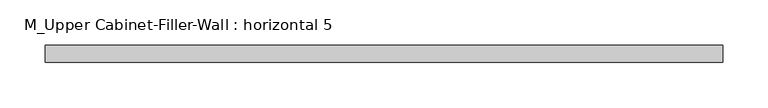
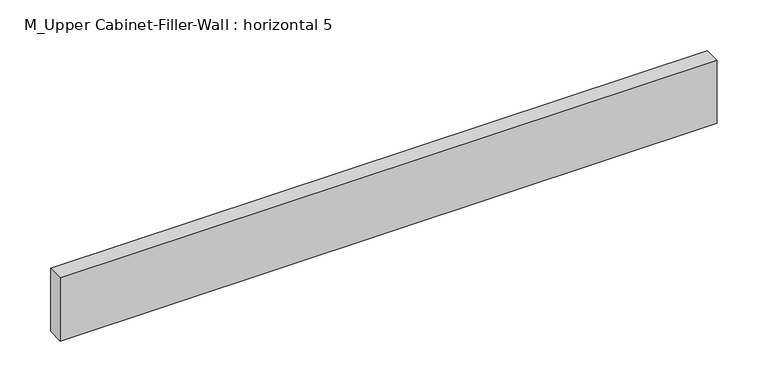
"""IFC4 building model written with IfcOpenShell, lengths in millimetres: furniture geometry, M_Upper Cabinet-Filler-Wall : horizontal 5."""

from ifc_helpers import new_model, si_unit, frame, origin, place, context, project, spatial, polyline, outline, extrude, source, transform, mapped, element, save


def m_upper_cabinet_filler_wall_horizontal_5_76bebc23(model_context):
    return source(origin(), model_context, "Body", "SweptSolid", [
        extrude(outline(polyline([(-344.8788372, 88.9), (-344.8788372, 107.95), (404.4211628, 107.95), (404.4211628, 88.9), (-344.8788372, 88.9)])), frame((0.0, 0.0, 1923.8), z_axis=(0.0, 0.0, 1.0), x_axis=(1.0, 0.0, 0.0)), (0.0, 0.0, 1.0), 76.2),
    ])


if __name__ == "__main__":
    model = new_model("IFC4")
    model_context = context("Model", 3, world=origin())
    ifc_project = project(units=[si_unit("LENGTHUNIT", "METRE", prefix="MILLI")], contexts=[model_context])
    site = spatial("IfcSite", under=ifc_project)
    building = spatial("IfcBuilding", under=site)
    placement = place(None, origin())
    m_upper_cabinet_filler_wall_horizontal_5_shape = m_upper_cabinet_filler_wall_horizontal_5_76bebc23(model_context)
    element("IfcFurniture", 1, ObjectType="M_Upper Cabinet-Filler-Wall : horizontal 5", at=placement, inside=building, context=model_context, shape_type="MappedRepresentation", body=[
        mapped(m_upper_cabinet_filler_wall_horizontal_5_shape, transform((0.0, 0.0, 0.0), x_axis=(1.0, 0.0, 0.0), y_axis=(0.0, 1.0, 0.0), z_axis=(0.0, 0.0, 1.0))),
    ])
    save(model, "model.ifc")

# Revit data of these elements
# Type "M_Upper Cabinet-Filler-Wall : horizontal 5"
#   Depth = 0' - 3"
#   Height = 0' - 3"
#   Top Of Cabinet = 6' - 6.74016"
#   Width = 2' - 5 1/2"
#   Cabinet Material = none
#   Default Elevation = 0
# Element 1 (IfcFurniture, "M_Upper Cabinet-Filler-Wall : horizontal 5")
#   Materials on its faces: "Cabinets"
# Materials
#   "Cabinets": class "Miscellaneous", colour RGB 249 249 249, transparency 0
